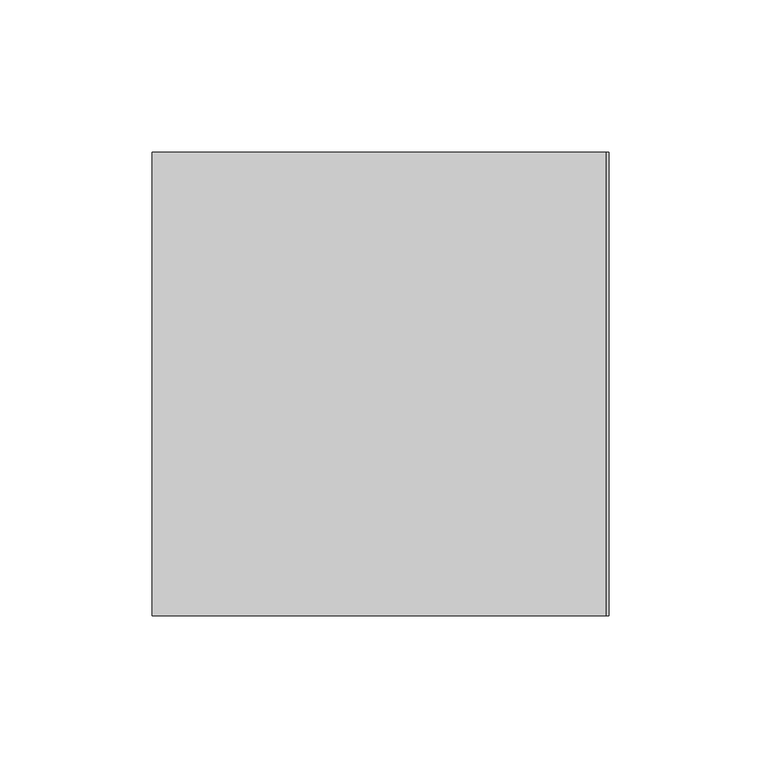
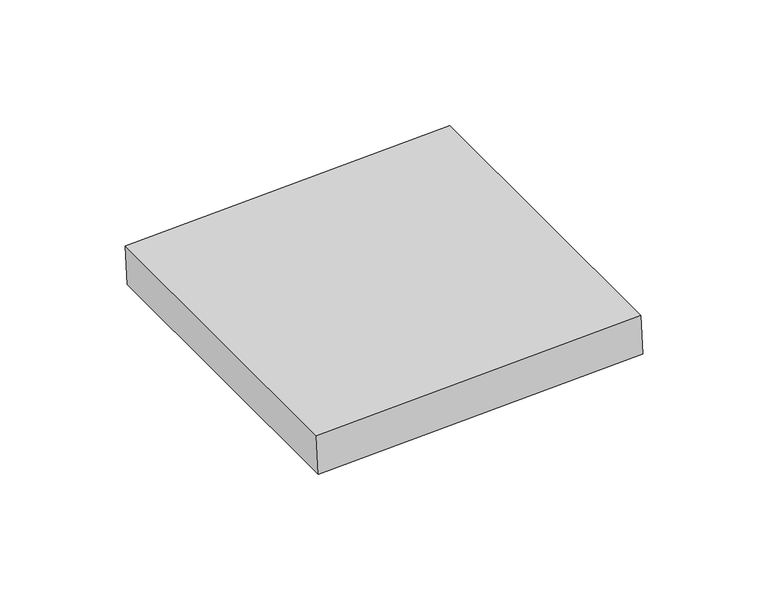
"""IFC4 building model written with IfcOpenShell, lengths in millimetres: proxy geometry, Generic Models 7:Generic Models 1:8:Generic Models 1:8 : Generic Models 7:Generic Models 1:337419:49 : Generic Models 7:Generic Models 1:8:Generic Models 1:8 : Generic Models 7:Generic Models 1:337419:315935."""

from ifc_helpers import new_model, si_unit, frame, origin, place, context, project, spatial, polyline, outline, extrude, source, transform, mapped, element, save


def generic_models_6fc7e062(model_context):
    return source(origin(), model_context, "Body", "SweptSolid", [
        extrude(outline(polyline([(0.0, -149.5247599), (0.0, 0.0), (152.4, 0.0), (152.4, -149.5247599), (0.0, -149.5247599)])), frame((560749.3638716, -578260.4833448, 3686.2435114), z_axis=(-0.04163054483311052, 0.0, 0.9991330730873133), x_axis=(0.0, -1.0, 0.0)), (0.0, 0.0, 1.0), 19.05),
    ])


if __name__ == "__main__":
    model = new_model("IFC4")
    model_context = context("Model", 3, world=origin())
    ifc_project = project(units=[si_unit("LENGTHUNIT", "METRE", prefix="MILLI")], contexts=[model_context])
    site = spatial("IfcSite", under=ifc_project)
    building = spatial("IfcBuilding", under=site)
    placement = place(None, origin())
    generic_models_shape = generic_models_6fc7e062(model_context)
    element("IfcBuildingElementProxy", 1, Name="Generic Models 7:Generic Models 1:8:Generic Models 1:8 : Generic Models 7:Generic Models 1:337419:49 : Generic Models 7:Generic Models 1:8:Generic Models 1:8 : Generic Models 7:Generic Models 1:337419:315935", ObjectType="Generic Models 7:Generic Models 1:8:Generic Models 1:8 : Generic Models 7:Generic Models 1:337419:49 : Generic Models 7:Generic Models 1:8:Generic Models 1:8 : Generic Models 7:Generic Models 1:337419:315935", at=placement, inside=building, context=model_context, shape_type="MappedRepresentation", body=[
        mapped(generic_models_shape, transform((0.0, 0.0, 0.0), x_axis=(1.0, 0.0, 0.0), y_axis=(0.0, 1.0, 0.0), z_axis=(0.0, 0.0, 1.0))),
    ])
    save(model, "model.ifc")

# Revit data of these elements
# Type "Generic Models 7:Generic Models 1:8:Generic Models 1:8 : Generic Models 7:Generic Models 1:337419:49 : Generic Models 7:Generic Models 1:8:Generic Models 1:8 : Generic Models 7:Generic Models 1:337419:315935"
#   NameOverride = "Generic Models 7:Generic Models 1:8:Generic Models 1:8 : Generic Models 7:Generic Models 1:337419:315935"
#   ObjectTypeOverride = "Generic Models 1:8 : Generic Models 7:Generic Models 1:337419"
#   Reference = "Generic Models 1"
#   Tag = "315935"
# Element 1 (IfcBuildingElementProxy, "Generic Models 7:Generic Models 1:8:Generic Models 1:8 : Generic Models 7:Generic Models 1:337419:49 : Generic Models 7:Generic Models 1:8:Generic Models 1:8 : Generic Models 7:Generic Models 1:337419:315935")
#   Materials on its faces: "LOW CONDUCTIVITY THERMAL BREAK PLATE"
# Materials
#   "LOW CONDUCTIVITY THERMAL BREAK PLATE": class "Generic", colour RGB 120 120 120, transparency 0, Cost = 0
